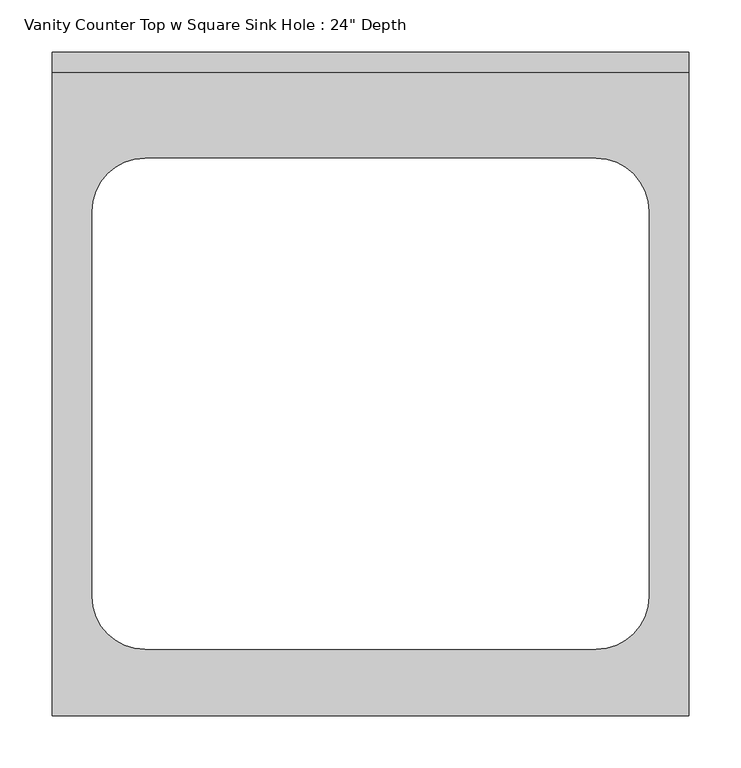
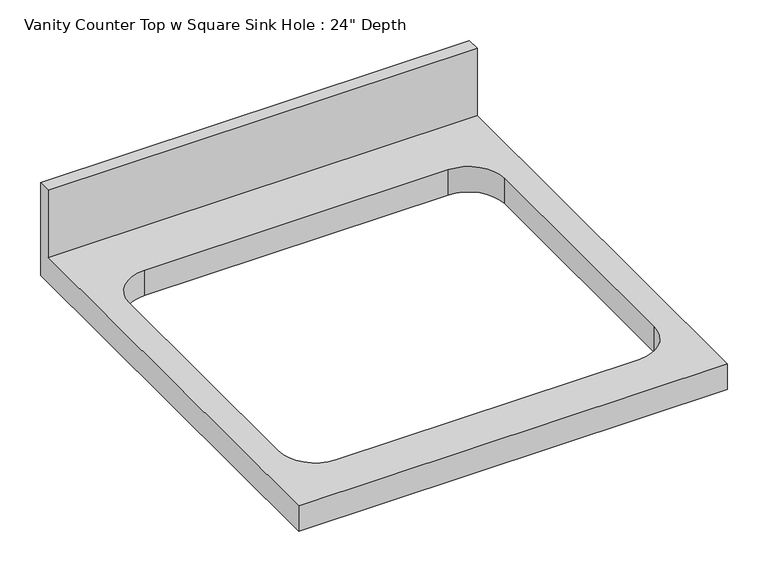
"""IFC4 building model written with IfcOpenShell, lengths in millimetres: furniture geometry."""

import ifcopenshell
import ifcopenshell.guid

model = None  # the IFC model being written
_history = None  # IfcOwnerHistory: only IFC2X3 demands one
_inside = {}  # id of a spatial element -> (the spatial element, [elements in it])
_under = {}  # id of a project, library or spatial element -> (it, [spatial elements below it])
_declared = {}  # id of a project -> (the project, [libraries it declares])
_typed = {}  # id of a type object -> (the type object, [elements of that type])
_made_of = {}  # id of a material, layer set ... -> (it, [elements and type objects made of it])


def new_model(schema):
    """Start an empty IFC model of exactly this schema.

    Asked for "IFC4X3", IfcOpenShell would pick the latest addendum, in which some entities
    have other attributes; the version numbers below select the first issue.
    IFC2X3 requires an IfcOwnerHistory on every rooted entity: one is made here for all.
    """
    global model, _history
    if schema == "IFC4X3":
        model = ifcopenshell.file(schema_version=(4, 3, 0, 0))
    else:
        model = ifcopenshell.file(schema=schema)
    _inside.clear()
    _under.clear()
    _declared.clear()
    _typed.clear()
    _made_of.clear()
    _history = None
    if model.schema == "IFC2X3":
        org = make("IfcOrganization", Name="unknown")
        user = make(
            "IfcPersonAndOrganization",
            ThePerson=make("IfcPerson", FamilyName="unknown"),
            TheOrganization=org,
        )
        app = make(
            "IfcApplication",
            ApplicationDeveloper=org,
            Version="unknown",
            ApplicationFullName="unknown",
            ApplicationIdentifier="unknown",
        )
        _history = make(
            "IfcOwnerHistory",
            OwningUser=user,
            OwningApplication=app,
            ChangeAction="ADDED",
            CreationDate=0,
        )
    return model


def make(cls, **values):
    """One entity of the class cls with the attributes given. An attribute that is None is left unset."""
    return model.create_entity(
        cls, **{name: value for name, value in values.items() if value is not None}
    )


def rooted(cls, **values):
    """An entity with a GlobalId (a new one), such as an element, a storey or a relation."""
    return make(cls, GlobalId=ifcopenshell.guid.new(), OwnerHistory=_history, **values)


def si_unit(unit_type, name, prefix=None):
    """IfcSIUnit, for example si_unit("LENGTHUNIT", "METRE", prefix="MILLI")."""
    return make("IfcSIUnit", UnitType=unit_type, Prefix=prefix, Name=name)


def assignment(units):
    """IfcUnitAssignment: the units of a project."""
    return None if units is None else make("IfcUnitAssignment", Units=units)


def point(xyz):
    """IfcCartesianPoint."""
    return None if xyz is None else make("IfcCartesianPoint", Coordinates=xyz)


def direction(xyz):
    """IfcDirection."""
    return None if xyz is None else make("IfcDirection", DirectionRatios=xyz)


def frame(location, z_axis=None, x_axis=None):
    """IfcAxis2Placement3D, a coordinate frame: its origin and axes. An axis left out is left unset."""
    return make(
        "IfcAxis2Placement3D",
        Location=point(location),
        Axis=direction(z_axis),
        RefDirection=direction(x_axis),
    )


def origin():
    """The frame at (0, 0, 0) with its axes left unset."""
    return frame((0.0, 0.0, 0.0))


def place(relative_to, where):
    """IfcLocalPlacement: puts the frame where relative to a parent placement (None: the world)."""
    return make(
        "IfcLocalPlacement", PlacementRelTo=relative_to, RelativePlacement=where
    )


def context(
    kind, dimensions, precision=None, world=None, true_north=None, identifier=None
):
    """IfcGeometricRepresentationContext, for example the 3D "Model" context."""
    return make(
        "IfcGeometricRepresentationContext",
        ContextIdentifier=identifier,
        ContextType=kind,
        CoordinateSpaceDimension=dimensions,
        Precision=precision,
        WorldCoordinateSystem=world,
        TrueNorth=true_north,
    )


def project(units=None, contexts=None):
    """IfcProject with its units and contexts."""
    return rooted(
        "IfcProject",
        Name="project",
        RepresentationContexts=contexts,
        UnitsInContext=assignment(units),
    )


def spatial(cls, under=None, at=None, **own):
    """A site, building, storey or space (cls), placed at a placement, below another one or the project."""
    s = rooted(cls, ObjectPlacement=at, **own)
    if under is not None:
        _under.setdefault(under.id(), (under, []))[1].append(s)
    return s


def polyline(points):
    """IfcPolyline through the points."""
    return make("IfcPolyline", Points=[point(p) for p in points])


def circle_curve(where, radius):
    """IfcCircle in the frame where."""
    return make("IfcCircle", Position=where, Radius=radius)


def shape(context_of_items, identifier, shape_type, items):
    """IfcShapeRepresentation: the items that make up one representation, for example the "Body"."""
    return make(
        "IfcShapeRepresentation",
        ContextOfItems=context_of_items,
        RepresentationIdentifier=identifier,
        RepresentationType=shape_type,
        Items=items,
    )


def source(mapping_origin, context_of_items, identifier, shape_type, items):
    """IfcRepresentationMap: a shape defined once, which mapped items show again and again."""
    return make(
        "IfcRepresentationMap",
        MappingOrigin=mapping_origin,
        MappedRepresentation=shape(context_of_items, identifier, shape_type, items),
    )


def transform(
    local_origin,
    x_axis=None,
    y_axis=None,
    z_axis=None,
    scale=None,
    scale2=None,
    scale3=None,
    uniform=True,
):
    """IfcCartesianTransformationOperator3D, or its non-uniform kind. x_axis, y_axis, z_axis: its Axis1, 2, 3."""
    if uniform:
        return make(
            "IfcCartesianTransformationOperator3D",
            Axis1=direction(x_axis),
            Axis2=direction(y_axis),
            LocalOrigin=point(local_origin),
            Scale=scale,
            Axis3=direction(z_axis),
        )
    return make(
        "IfcCartesianTransformationOperator3DnonUniform",
        Axis1=direction(x_axis),
        Axis2=direction(y_axis),
        LocalOrigin=point(local_origin),
        Scale=scale,
        Axis3=direction(z_axis),
        Scale2=scale2,
        Scale3=scale3,
    )


def mapped(mapping_source, mapping_target):
    """IfcMappedItem: shows the shape of a source again, moved by a transform."""
    return make(
        "IfcMappedItem", MappingSource=mapping_source, MappingTarget=mapping_target
    )


def made_of(thing, what):
    """Note that an element or type object is made of a material, layer set ...; save() writes the relation."""
    if what is not None:
        _made_of.setdefault(what.id(), (what, []))[1].append(thing)
    return thing


def element(
    cls,
    number,
    at=None,
    inside=None,
    cuts=None,
    type_object=None,
    material=None,
    context=None,
    identifier="Body",
    shape_type=None,
    held_by="IfcProductDefinitionShape",
    body=None,
    shapes=None,
    **own,
):
    """One element of the class cls, such as IfcWall. Its Tag is "e" and its number.

    at: its placement. inside: the storey or other place that contains it. cuts: it is an
    opening in that element (IfcRelVoidsElement). A single representation is given by context,
    identifier, shape_type and body (its items); several are given by shapes. held_by: the class
    of the entity that holds the representations. save() writes the other relations.
    """
    e = rooted(cls, Tag="e%d" % number, ObjectPlacement=at, **own)
    if body is not None:
        shapes = [shape(context, identifier, shape_type, body)]
    if shapes is not None:
        e.Representation = make(held_by, Representations=shapes)
    if inside is not None:
        _inside.setdefault(inside.id(), (inside, []))[1].append(e)
    if cuts is not None:
        rooted(
            "IfcRelVoidsElement", RelatingBuildingElement=cuts, RelatedOpeningElement=e
        )
    if type_object is not None:
        _typed.setdefault(type_object.id(), (type_object, []))[1].append(e)
    return made_of(e, material)


def aggregate(whole, parts):
    """IfcRelAggregates: a whole, such as a stair, and the parts it consists of."""
    return rooted("IfcRelAggregates", RelatingObject=whole, RelatedObjects=parts)


def save(model, path):
    """Write the relations noted so far, then the file.

    IfcRelAggregates (storeys below a building ...), IfcRelContainedInSpatialStructure (elements
    in a storey), IfcRelDefinesByType, IfcRelAssociatesMaterial and IfcRelDeclares: one each for
    every whole, place, type object, material and project.
    """
    for whole, parts in _under.values():
        aggregate(whole, parts)
    for where, things in _inside.values():
        rooted(
            "IfcRelContainedInSpatialStructure",
            RelatedElements=things,
            RelatingStructure=where,
        )
    for kind, things in _typed.values():
        rooted("IfcRelDefinesByType", RelatedObjects=things, RelatingType=kind)
    for what, things in _made_of.values():
        rooted("IfcRelAssociatesMaterial", RelatedObjects=things, RelatingMaterial=what)
    for by, libraries in _declared.values():
        rooted("IfcRelDeclares", RelatingContext=by, RelatedDefinitions=libraries)
    model.write(path)


def plane_surface(at):
    """IfcPlane: the flat surface through the origin of the frame at, square to its z axis."""
    return make("IfcPlane", Position=at)


def revolved_surface(curve, axis_point, axis_direction):
    """IfcSurfaceOfRevolution: the curve turned about the line through axis_point along axis_direction."""
    return make(
        "IfcSurfaceOfRevolution",
        SweptCurve=make("IfcArbitraryOpenProfileDef", ProfileType="CURVE", Curve=curve),
        AxisPosition=make("IfcAxis1Placement", Location=point(axis_point), Axis=direction(axis_direction)),
    )


def advanced_brep(points, edges, surfaces, faces):
    """IfcAdvancedBrep: a solid bounded by faces that lie on surfaces and meet in shared edges.

    An edge is (start, end): straight between two places in points (the first is 0);
    or (start, end, curve); or (start, end, curve, False) where it runs against its curve.
    A face is (place in surfaces, loops), or (place, loops, False) where it looks against
    its surface's normal. A loop lists edges by number (the first is 1), with a minus sign
    where the edge is run from its end to its start. The first loop is the outer one.
    """
    corners = [point(p) for p in points]
    vertices = [make("IfcVertexPoint", VertexGeometry=c) for c in corners]
    made = []
    for start, end, *more in edges:
        made.append(
            make(
                "IfcEdgeCurve",
                EdgeStart=vertices[start],
                EdgeEnd=vertices[end],
                EdgeGeometry=more[0] if more else make("IfcPolyline", Points=[corners[start], corners[end]]),
                SameSense=more[1] if len(more) > 1 else True,
            )
        )
    hull = []
    for where, loops, *sense in faces:
        bounds = []
        for j, loop in enumerate(loops):
            ring = [make("IfcOrientedEdge", EdgeElement=made[abs(k) - 1], Orientation=k > 0) for k in loop]
            bounds.append(
                make(
                    "IfcFaceOuterBound" if j == 0 else "IfcFaceBound",
                    Bound=make("IfcEdgeLoop", EdgeList=ring),
                    Orientation=True,
                )
            )
        hull.append(make("IfcAdvancedFace", Bounds=bounds, FaceSurface=surfaces[where], SameSense=sense[0] if sense else True))
    return make("IfcAdvancedBrep", Outer=make("IfcClosedShell", CfsFaces=hull))


def furniture_9bca86e0(model_context):
    return source(origin(), model_context, "Body", "AdvancedBrep", [
        advanced_brep(
        [(-1268.7247951, -635.0, 787.4), (-659.1247951, -635.0, 787.4), (-659.1247951, -19.05, 787.4), (-1268.7247951, -19.05, 787.4), (-1230.6247951, -152.4, 787.4), (-1179.8247951, -101.6, 787.4), (-748.0247951, -101.6, 787.4), (-697.2247951, -152.4, 787.4), (-697.2247951, -520.7, 787.4), (-748.0247951, -571.5, 787.4), (-1179.8247951, -571.5, 787.4), (-1230.6247951, -520.7, 787.4), (-659.1247951, 0.0, 749.3), (-659.1247951, -635.0, 749.3), (-1268.7247951, -635.0, 749.3), (-1268.7247951, 0.0, 749.3), (-1179.8247951, -101.6, 749.3), (-1230.6247951, -152.4, 749.3), (-1230.6247951, -520.7, 749.3), (-1179.8247951, -571.5, 749.3), (-748.0247951, -571.5, 749.3), (-697.2247951, -520.7, 749.3), (-697.2247951, -152.4, 749.3), (-748.0247951, -101.6, 749.3), (-1268.7247951, 0.0, 889.0), (-659.1247951, 0.0, 889.0), (-1268.7247951, -19.05, 889.0), (-659.1247951, -19.05, 889.0)],
        [
            (0, 1),
            (1, 2),
            (2, 3),
            (3, 0),
            (4, 5, circle_curve(frame((-1179.8247951, -152.4, 787.4), z_axis=(0.0, 0.0, -1.0), x_axis=(1.0, 0.0, 0.0)), 50.8)),
            (5, 6),
            (6, 7, circle_curve(frame((-748.0247951, -152.4, 787.4), z_axis=(0.0, 0.0, -1.0), x_axis=(1.0, 0.0, 0.0)), 50.8)),
            (7, 8),
            (8, 9, circle_curve(frame((-748.0247951, -520.7, 787.4), z_axis=(0.0, 0.0, -1.0), x_axis=(1.0, 0.0, 0.0)), 50.8)),
            (9, 10),
            (10, 11, circle_curve(frame((-1179.8247951, -520.7, 787.4), z_axis=(0.0, 0.0, -1.0), x_axis=(1.0, 0.0, 0.0)), 50.8)),
            (11, 4),
            (12, 13),
            (13, 14),
            (14, 15),
            (15, 12),
            (16, 17, circle_curve(frame((-1179.8247951, -152.4, 749.3), z_axis=(0.0, 0.0, 1.0), x_axis=(1.0, 0.0, 0.0)), 50.8)),
            (17, 18),
            (18, 19, circle_curve(frame((-1179.8247951, -520.7, 749.3), z_axis=(0.0, 0.0, 1.0), x_axis=(1.0, 0.0, 0.0)), 50.8)),
            (19, 20),
            (20, 21, circle_curve(frame((-748.0247951, -520.7, 749.3), z_axis=(0.0, 0.0, 1.0), x_axis=(1.0, 0.0, 0.0)), 50.8)),
            (21, 22),
            (22, 23, circle_curve(frame((-748.0247951, -152.4, 749.3), z_axis=(0.0, 0.0, 1.0), x_axis=(1.0, 0.0, 0.0)), 50.8)),
            (23, 16),
            (15, 24),
            (24, 25),
            (25, 12),
            (14, 0),
            (3, 26),
            (26, 24),
            (13, 1),
            (25, 27),
            (27, 2),
            (26, 27),
            (4, 17),
            (16, 5),
            (11, 18),
            (10, 19),
            (9, 20),
            (8, 21),
            (7, 22),
            (6, 23),
        ],
        [
            plane_surface(frame((-1268.7247951, 0.0, 787.4), z_axis=(0.0, 0.0, 1.0), x_axis=(-1.0, 0.0, 0.0))),
            plane_surface(frame((-1268.7247951, 0.0, 749.3), z_axis=(0.0, 0.0, -1.0), x_axis=(1.0, 0.0, 0.0))),
            plane_surface(frame((-659.1247951, 0.0, 787.4), z_axis=(0.0, 1.0, 0.0), x_axis=(0.0, 0.0, -1.0))),
            plane_surface(frame((-1268.7247951, 0.0, 787.4), z_axis=(-1.0, 0.0, 0.0), x_axis=(0.0, 0.0, -1.0))),
            plane_surface(frame((-1268.7247951, -635.0, 787.4), z_axis=(0.0, -1.0, 0.0), x_axis=(0.0, 0.0, -1.0))),
            plane_surface(frame((-659.1247951, -635.0, 787.4), z_axis=(1.0, 0.0, 0.0), x_axis=(0.0, 0.0, -1.0))),
            plane_surface(frame((-1268.7247951, 0.0, 889.0), z_axis=(0.0, 0.0, 1.0), x_axis=(0.0, -1.0, 0.0))),
            plane_surface(frame((-1268.7247951, -19.05, 889.0), z_axis=(0.0, -1.0, 0.0), x_axis=(0.0, 0.0, -1.0))),
            revolved_surface(polyline([(-1129.0247951000001, -152.4, 787.4), (-1129.0247951000001, -152.4, 749.3)]), (-1179.8247951, -152.4, 749.3), (0.0, 0.0, 1.0)),
            plane_surface(frame((-1230.6247951, -152.4, 787.4), z_axis=(1.0, 0.0, 0.0), x_axis=(0.0, 0.0, -1.0))),
            revolved_surface(polyline([(-1129.0247951000001, -520.7, 787.4), (-1129.0247951000001, -520.7, 749.3)]), (-1179.8247951, -520.7, 749.3), (0.0, 0.0, 1.0)),
            plane_surface(frame((-1179.8247951, -571.5, 787.4), z_axis=(0.0, 1.0, 0.0), x_axis=(0.0, 0.0, -1.0))),
            revolved_surface(polyline([(-697.2247951, -520.7, 787.4), (-697.2247951, -520.7, 749.3)]), (-748.0247951, -520.7, 749.3), (0.0, 0.0, 1.0)),
            plane_surface(frame((-697.2247951, -520.7, 787.4), z_axis=(-1.0, 0.0, 0.0), x_axis=(0.0, 0.0, -1.0))),
            revolved_surface(polyline([(-697.2247951, -152.4, 787.4), (-697.2247951, -152.4, 749.3)]), (-748.0247951, -152.4, 749.3), (0.0, 0.0, 1.0)),
            plane_surface(frame((-748.0247951, -101.6, 787.4), z_axis=(0.0, -1.0, 0.0), x_axis=(0.0, 0.0, -1.0))),
        ],
        [
            (0, [[1, 2, 3, 4], [5, 6, 7, 8, 9, 10, 11, 12]]),
            (1, [[13, 14, 15, 16], [17, 18, 19, 20, 21, 22, 23, 24]]),
            (2, [[-16, 25, 26, 27]]),
            (3, [[-15, 28, -4, 29, 30, -25]]),
            (4, [[-1, -28, -14, 31]]),
            (5, [[-13, -27, 32, 33, -2, -31]]),
            (6, [[-30, 34, -32, -26]]),
            (7, [[-34, -29, -3, -33]]),
            (8, [[35, -17, 36, -5]]),
            (9, [[-35, -12, 37, -18]]),
            (10, [[-37, -11, 38, -19]]),
            (11, [[-38, -10, 39, -20]]),
            (12, [[-39, -9, 40, -21]]),
            (13, [[-40, -8, 41, -22]]),
            (14, [[-41, -7, 42, -23]]),
            (15, [[-36, -24, -42, -6]]),
        ],
    ),
    ])


if __name__ == "__main__":
    model = new_model("IFC4")
    model_context = context("Model", 3, world=origin())
    ifc_project = project(units=[si_unit("LENGTHUNIT", "METRE", prefix="MILLI")], contexts=[model_context])
    site = spatial("IfcSite", under=ifc_project)
    building = spatial("IfcBuilding", under=site)
    placement = place(None, origin())
    furniture_shape = furniture_9bca86e0(model_context)
    element("IfcFurniture", 1, ObjectType="Vanity Counter Top w Square Sink Hole : 24\" Depth", at=placement, inside=building, context=model_context, shape_type="MappedRepresentation", body=[
        mapped(furniture_shape, transform((0.0, 0.0, 0.0), x_axis=(1.0, 0.0, 0.0), y_axis=(0.0, 1.0, 0.0), z_axis=(0.0, 0.0, 1.0))),
    ])
    save(model, "model.ifc")

# Revit data of these elements
# Type "Vanity Counter Top w Square Sink Hole : 24\" Depth"
#   Assembly Code = "C1030400"
#   Counter Thickness = 0' - 1 1/2"
#   Depth = 2' - 1"
#   Height = 2' - 7"
#   Length [instance default] = 4' - 0"
#   Sink Location [instance default] = 2' - 0"
#   Sink Location To Wall [instance default] = 0' - 4 1/2"
#   Sink Opening Depth [instance default] = 1' - 5 1/2"
#   Sink Opening Width [instance default] = 1' - 8"
#   Counter Top Material = none
# Element 1 (IfcFurniture, "Vanity Counter Top w Square Sink Hole : 24\" Depth")
#   Length = 2' - 0"
#   Sink Location = 1' - 0"
#   Materials on its faces: "Counter Top"
# Materials
#   "Counter Top": class "Wood", colour RGB 226 177 128, transparency 0
